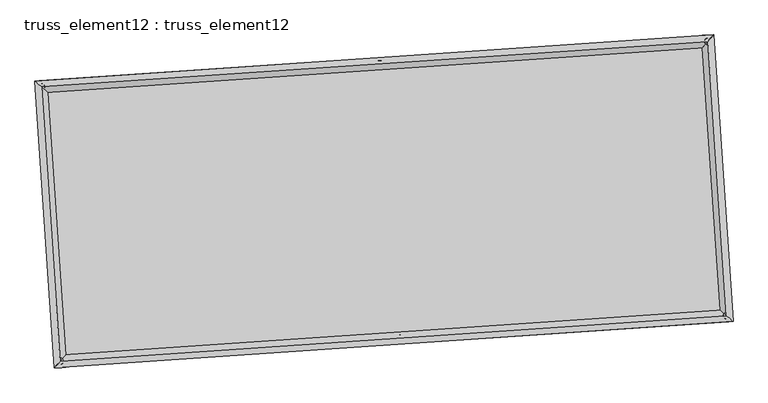
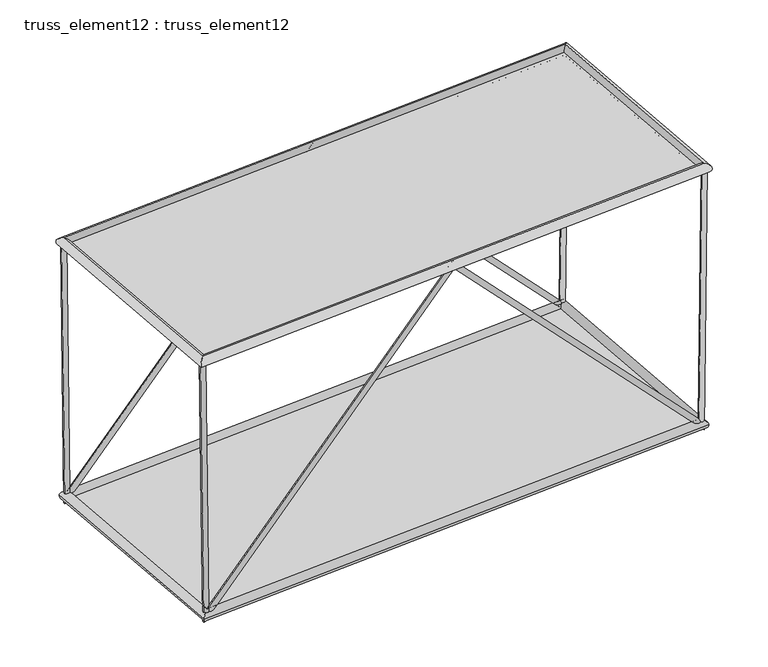
"""IFC4 building model written with IfcOpenShell, lengths in millimetres: plate geometry, truss_element12 : truss_element12."""

import ifcopenshell
import ifcopenshell.guid

model = None  # the IFC model being written
_history = None  # IfcOwnerHistory: only IFC2X3 demands one
_inside = {}  # id of a spatial element -> (the spatial element, [elements in it])
_under = {}  # id of a project, library or spatial element -> (it, [spatial elements below it])
_declared = {}  # id of a project -> (the project, [libraries it declares])
_typed = {}  # id of a type object -> (the type object, [elements of that type])
_made_of = {}  # id of a material, layer set ... -> (it, [elements and type objects made of it])


def new_model(schema):
    """Start an empty IFC model of exactly this schema.

    Asked for "IFC4X3", IfcOpenShell would pick the latest addendum, in which some entities
    have other attributes; the version numbers below select the first issue.
    IFC2X3 requires an IfcOwnerHistory on every rooted entity: one is made here for all.
    """
    global model, _history
    if schema == "IFC4X3":
        model = ifcopenshell.file(schema_version=(4, 3, 0, 0))
    else:
        model = ifcopenshell.file(schema=schema)
    _inside.clear()
    _under.clear()
    _declared.clear()
    _typed.clear()
    _made_of.clear()
    _history = None
    if model.schema == "IFC2X3":
        org = make("IfcOrganization", Name="unknown")
        user = make(
            "IfcPersonAndOrganization",
            ThePerson=make("IfcPerson", FamilyName="unknown"),
            TheOrganization=org,
        )
        app = make(
            "IfcApplication",
            ApplicationDeveloper=org,
            Version="unknown",
            ApplicationFullName="unknown",
            ApplicationIdentifier="unknown",
        )
        _history = make(
            "IfcOwnerHistory",
            OwningUser=user,
            OwningApplication=app,
            ChangeAction="ADDED",
            CreationDate=0,
        )
    return model


def make(cls, **values):
    """One entity of the class cls with the attributes given. An attribute that is None is left unset."""
    return model.create_entity(
        cls, **{name: value for name, value in values.items() if value is not None}
    )


def rooted(cls, **values):
    """An entity with a GlobalId (a new one), such as an element, a storey or a relation."""
    return make(cls, GlobalId=ifcopenshell.guid.new(), OwnerHistory=_history, **values)


def si_unit(unit_type, name, prefix=None):
    """IfcSIUnit, for example si_unit("LENGTHUNIT", "METRE", prefix="MILLI")."""
    return make("IfcSIUnit", UnitType=unit_type, Prefix=prefix, Name=name)


def assignment(units):
    """IfcUnitAssignment: the units of a project."""
    return None if units is None else make("IfcUnitAssignment", Units=units)


def point(xyz):
    """IfcCartesianPoint."""
    return None if xyz is None else make("IfcCartesianPoint", Coordinates=xyz)


def direction(xyz):
    """IfcDirection."""
    return None if xyz is None else make("IfcDirection", DirectionRatios=xyz)


def frame(location, z_axis=None, x_axis=None):
    """IfcAxis2Placement3D, a coordinate frame: its origin and axes. An axis left out is left unset."""
    return make(
        "IfcAxis2Placement3D",
        Location=point(location),
        Axis=direction(z_axis),
        RefDirection=direction(x_axis),
    )


def origin():
    """The frame at (0, 0, 0) with its axes left unset."""
    return frame((0.0, 0.0, 0.0))


def origin_with_axes():
    """The frame at (0, 0, 0) with the z axis (0, 0, 1) and the x axis (1, 0, 0) written out."""
    return frame((0.0, 0.0, 0.0), z_axis=(0.0, 0.0, 1.0), x_axis=(1.0, 0.0, 0.0))


def place(relative_to, where):
    """IfcLocalPlacement: puts the frame where relative to a parent placement (None: the world)."""
    return make(
        "IfcLocalPlacement", PlacementRelTo=relative_to, RelativePlacement=where
    )


def context(
    kind, dimensions, precision=None, world=None, true_north=None, identifier=None
):
    """IfcGeometricRepresentationContext, for example the 3D "Model" context."""
    return make(
        "IfcGeometricRepresentationContext",
        ContextIdentifier=identifier,
        ContextType=kind,
        CoordinateSpaceDimension=dimensions,
        Precision=precision,
        WorldCoordinateSystem=world,
        TrueNorth=true_north,
    )


def project(units=None, contexts=None):
    """IfcProject with its units and contexts."""
    return rooted(
        "IfcProject",
        Name="project",
        RepresentationContexts=contexts,
        UnitsInContext=assignment(units),
    )


def spatial(cls, under=None, at=None, **own):
    """A site, building, storey or space (cls), placed at a placement, below another one or the project."""
    s = rooted(cls, ObjectPlacement=at, **own)
    if under is not None:
        _under.setdefault(under.id(), (under, []))[1].append(s)
    return s


def polyline(points):
    """IfcPolyline through the points."""
    return make("IfcPolyline", Points=[point(p) for p in points])


def circle_curve(where, radius):
    """IfcCircle in the frame where."""
    return make("IfcCircle", Position=where, Radius=radius)


def ellipse_curve(where, semi_axis1, semi_axis2):
    """IfcEllipse in the frame where."""
    return make(
        "IfcEllipse", Position=where, SemiAxis1=semi_axis1, SemiAxis2=semi_axis2
    )


def outline(outer, holes=None, kind="AREA"):
    """IfcArbitraryClosedProfileDef: a profile drawn as a closed curve; with holes, ...WithVoids."""
    if holes is None:
        return make("IfcArbitraryClosedProfileDef", ProfileType=kind, OuterCurve=outer)
    return make(
        "IfcArbitraryProfileDefWithVoids",
        ProfileType=kind,
        OuterCurve=outer,
        InnerCurves=holes,
    )


def extrude(swept, where, along, depth):
    """IfcExtrudedAreaSolid: the profile swept, set in the frame where, extruded along a direction by depth."""
    return make(
        "IfcExtrudedAreaSolid",
        SweptArea=swept,
        Position=where,
        ExtrudedDirection=direction(along),
        Depth=depth,
    )


def shape(context_of_items, identifier, shape_type, items):
    """IfcShapeRepresentation: the items that make up one representation, for example the "Body"."""
    return make(
        "IfcShapeRepresentation",
        ContextOfItems=context_of_items,
        RepresentationIdentifier=identifier,
        RepresentationType=shape_type,
        Items=items,
    )


def source(mapping_origin, context_of_items, identifier, shape_type, items):
    """IfcRepresentationMap: a shape defined once, which mapped items show again and again."""
    return make(
        "IfcRepresentationMap",
        MappingOrigin=mapping_origin,
        MappedRepresentation=shape(context_of_items, identifier, shape_type, items),
    )


def transform(
    local_origin,
    x_axis=None,
    y_axis=None,
    z_axis=None,
    scale=None,
    scale2=None,
    scale3=None,
    uniform=True,
):
    """IfcCartesianTransformationOperator3D, or its non-uniform kind. x_axis, y_axis, z_axis: its Axis1, 2, 3."""
    if uniform:
        return make(
            "IfcCartesianTransformationOperator3D",
            Axis1=direction(x_axis),
            Axis2=direction(y_axis),
            LocalOrigin=point(local_origin),
            Scale=scale,
            Axis3=direction(z_axis),
        )
    return make(
        "IfcCartesianTransformationOperator3DnonUniform",
        Axis1=direction(x_axis),
        Axis2=direction(y_axis),
        LocalOrigin=point(local_origin),
        Scale=scale,
        Axis3=direction(z_axis),
        Scale2=scale2,
        Scale3=scale3,
    )


def mapped(mapping_source, mapping_target):
    """IfcMappedItem: shows the shape of a source again, moved by a transform."""
    return make(
        "IfcMappedItem", MappingSource=mapping_source, MappingTarget=mapping_target
    )


def made_of(thing, what):
    """Note that an element or type object is made of a material, layer set ...; save() writes the relation."""
    if what is not None:
        _made_of.setdefault(what.id(), (what, []))[1].append(thing)
    return thing


def element(
    cls,
    number,
    at=None,
    inside=None,
    cuts=None,
    type_object=None,
    material=None,
    context=None,
    identifier="Body",
    shape_type=None,
    held_by="IfcProductDefinitionShape",
    body=None,
    shapes=None,
    **own,
):
    """One element of the class cls, such as IfcWall. Its Tag is "e" and its number.

    at: its placement. inside: the storey or other place that contains it. cuts: it is an
    opening in that element (IfcRelVoidsElement). A single representation is given by context,
    identifier, shape_type and body (its items); several are given by shapes. held_by: the class
    of the entity that holds the representations. save() writes the other relations.
    """
    e = rooted(cls, Tag="e%d" % number, ObjectPlacement=at, **own)
    if body is not None:
        shapes = [shape(context, identifier, shape_type, body)]
    if shapes is not None:
        e.Representation = make(held_by, Representations=shapes)
    if inside is not None:
        _inside.setdefault(inside.id(), (inside, []))[1].append(e)
    if cuts is not None:
        rooted(
            "IfcRelVoidsElement", RelatingBuildingElement=cuts, RelatedOpeningElement=e
        )
    if type_object is not None:
        _typed.setdefault(type_object.id(), (type_object, []))[1].append(e)
    return made_of(e, material)


def aggregate(whole, parts):
    """IfcRelAggregates: a whole, such as a stair, and the parts it consists of."""
    return rooted("IfcRelAggregates", RelatingObject=whole, RelatedObjects=parts)


def save(model, path):
    """Write the relations noted so far, then the file.

    IfcRelAggregates (storeys below a building ...), IfcRelContainedInSpatialStructure (elements
    in a storey), IfcRelDefinesByType, IfcRelAssociatesMaterial and IfcRelDeclares: one each for
    every whole, place, type object, material and project.
    """
    for whole, parts in _under.values():
        aggregate(whole, parts)
    for where, things in _inside.values():
        rooted(
            "IfcRelContainedInSpatialStructure",
            RelatedElements=things,
            RelatingStructure=where,
        )
    for kind, things in _typed.values():
        rooted("IfcRelDefinesByType", RelatedObjects=things, RelatingType=kind)
    for what, things in _made_of.values():
        rooted("IfcRelAssociatesMaterial", RelatedObjects=things, RelatingMaterial=what)
    for by, libraries in _declared.values():
        rooted("IfcRelDeclares", RelatingContext=by, RelatedDefinitions=libraries)
    model.write(path)


def plane_surface(at):
    """IfcPlane: the flat surface through the origin of the frame at, square to its z axis."""
    return make("IfcPlane", Position=at)


def cylinder_surface(at, radius):
    """IfcCylindricalSurface: all points at the distance radius from the z axis of the frame at."""
    return make("IfcCylindricalSurface", Position=at, Radius=radius)


def advanced_brep(points, edges, surfaces, faces):
    """IfcAdvancedBrep: a solid bounded by faces that lie on surfaces and meet in shared edges.

    An edge is (start, end): straight between two places in points (the first is 0);
    or (start, end, curve); or (start, end, curve, False) where it runs against its curve.
    A face is (place in surfaces, loops), or (place, loops, False) where it looks against
    its surface's normal. A loop lists edges by number (the first is 1), with a minus sign
    where the edge is run from its end to its start. The first loop is the outer one.
    """
    corners = [point(p) for p in points]
    vertices = [make("IfcVertexPoint", VertexGeometry=c) for c in corners]
    made = []
    for start, end, *more in edges:
        made.append(
            make(
                "IfcEdgeCurve",
                EdgeStart=vertices[start],
                EdgeEnd=vertices[end],
                EdgeGeometry=more[0] if more else make("IfcPolyline", Points=[corners[start], corners[end]]),
                SameSense=more[1] if len(more) > 1 else True,
            )
        )
    hull = []
    for where, loops, *sense in faces:
        bounds = []
        for j, loop in enumerate(loops):
            ring = [make("IfcOrientedEdge", EdgeElement=made[abs(k) - 1], Orientation=k > 0) for k in loop]
            bounds.append(
                make(
                    "IfcFaceOuterBound" if j == 0 else "IfcFaceBound",
                    Bound=make("IfcEdgeLoop", EdgeList=ring),
                    Orientation=True,
                )
            )
        hull.append(make("IfcAdvancedFace", Bounds=bounds, FaceSurface=surfaces[where], SameSense=sense[0] if sense else True))
    return make("IfcAdvancedBrep", Outer=make("IfcClosedShell", CfsFaces=hull))


def truss_element12_truss_element12_2c86acb7(model_context):
    return source(origin(), model_context, "Body", "SolidModel", [
        advanced_brep(
        [(-3728.3550112, 2271.9000693, 5000.230225), (-3827.45033, 2258.5393422, 4998.9618576), (-3666.4925131, 2276.1182379, 122.5885244), (-3762.4943697, 2262.9684422, -122.5885244), (1063.1473442, 2598.6144007, 5071.7241818), (1063.6040901, 2592.0417504, 4927.4822409), (5793.903749, 2921.1866967, 122.5964773), (5890.857228, 2921.1937918, -122.5964773), (5854.658099, 2925.3293049, 5000.2332074), (5954.6501108, 2925.543586, 4998.9875555)],
        [
            (0, 1, circle_curve(frame((-3777.9026706, 2265.2197058, 4999.5960413), z_axis=(-0.012681845830498275, -0.0008647268589742656, 0.9999192082532422), x_axis=(-0.13360744533254773, 0.991033979828119, -0.0008374829847137765)), 50.0)),
            (1, 0, circle_curve(frame((-3777.9026706, 2265.2197058, 4999.5960413), z_axis=(-0.012681845830498275, -0.0008647268589742656, 0.9999192082532422), x_axis=(-0.13360744533254773, 0.991033979828119, -0.0008374829847137765)), 50.0)),
            (0, 2),
            (2, 3, ellipse_curve(frame((-3714.4934414, 2269.54334, 0.0), z_axis=(-0.9281379125811652, -0.06328619607639939, 0.3668172196280557), x_axis=(0.36596744941726267, 0.02495392920324594, 0.9302930330730971)), 132.0610358, 50.0)),
            (3, 1),
            (3, 2, ellipse_curve(frame((-3714.4934414, 2269.54334, 0.0), z_axis=(-0.9281379125811652, -0.06328619607639939, 0.3668172196280557), x_axis=(0.36596744941726267, 0.02495392920324594, 0.9302930330730971)), 132.0610358, 50.0)),
            (2, 4),
            (4, 5, ellipse_curve(frame((1063.3757172, 2595.3280756, 4999.6032114), z_axis=(-0.99768339431723, -0.068028238108855, -5.9358703528731525e-05), x_axis=(5.922119292306359e-05, 4.038068026292035e-06, -0.9999999982382721)), 72.2780144, 50.0)),
            (5, 3),
            (5, 4, ellipse_curve(frame((1063.3757172, 2595.3280756, 4999.6032114), z_axis=(-0.99768339431723, -0.068028238108855, -5.9358703528731525e-05), x_axis=(5.922119292306359e-05, 4.038068026292035e-06, -0.9999999982382721)), 72.2780144, 50.0)),
            (4, 6),
            (6, 7, ellipse_curve(frame((5842.3804885, 2921.1902443, 0.0), z_axis=(-0.9280745157714422, -0.06328187328893672, -0.3669783340861503), x_axis=(-0.3661281906369709, -0.02496488953598652, 0.9302294890570573)), 132.0786249, 50.0)),
            (7, 5),
            (7, 6, ellipse_curve(frame((5842.3804885, 2921.1902443, 0.0), z_axis=(-0.9280745157714422, -0.06328187328893672, -0.3669783340861503), x_axis=(-0.3661281906369709, -0.02496488953598652, 0.9302294890570573)), 132.0786249, 50.0)),
            (8, 9, circle_curve(frame((5904.6541049, 2925.4364454, 4999.6103815), z_axis=(0.012454723282468173, 0.0008492402357941579, 0.9999220762934375), x_axis=(-0.002153222592044798, 0.9999973435725115, -0.0008224842793232085)), 50.0)),
            (9, 8, circle_curve(frame((5904.6541049, 2925.4364454, 4999.6103815), z_axis=(0.012454723282468173, 0.0008492402357941579, 0.9999220762934375), x_axis=(-0.002153222592044798, 0.9999973435725115, -0.0008224842793232085)), 50.0)),
            (6, 8),
            (9, 7),
        ],
        [
            plane_surface(frame((-3777.9026706, 2315.2196871, 4999.6392811), z_axis=(-0.012681845830499536, -0.000864726858973905, 0.9999192082532424), x_axis=(0.9999195821596513, -1.0967214670642997e-05, 0.012681841088294742))),
            cylinder_surface(frame((-3777.9026706, 2265.2197058, 4999.5960413), z_axis=(-0.012681845830498278, -0.0008647268589742659, 0.9999192082532424), x_axis=(-0.13360744533254773, 0.991033979828119, -0.0008374829847137765)), 50.0),
            cylinder_surface(frame((-3714.4934414, 2269.54334, 0.0), z_axis=(-0.6901279623524452, -0.04705720233082468, -0.7221558109494499), x_axis=(-0.020411445780293115, 0.9987523847393089, -0.04557462955089897)), 50.0),
            cylinder_surface(frame((1063.3757172, 2595.3280756, 4999.6032114), z_axis=(-0.6902134913462256, -0.04706303422778687, 0.7220736854178583), x_axis=(-0.11534401236489931, 0.9922792938963748, -0.04558027770953044)), 50.0),
            plane_surface(frame((5904.6541049, 2875.4364635, 4999.6528468), z_axis=(0.012454723282466664, 0.0008492402357928526, 0.9999220762934377), x_axis=(0.9999224369259634, -1.0577872590289415e-05, -0.012454718790539939))),
            cylinder_surface(frame((5842.3804885, 2921.1902443, 0.0), z_axis=(-0.012454723282468173, -0.0008492402357941579, -0.9999220762934375), x_axis=(-0.002153222592044798, 0.9999973435725115, -0.0008224842793232085)), 50.0),
        ],
        [
            (0, [[1, 2]]),
            (1, [[-1, 3, 4, 5]]),
            (1, [[-2, -5, 6, -3]]),
            (2, [[-4, 7, 8, 9]]),
            (2, [[-6, -9, 10, -7]]),
            (3, [[-8, 11, 12, 13]]),
            (3, [[-10, -13, 14, -11]]),
            (4, [[15, 16]]),
            (5, [[-12, 17, -16, 18]]),
            (5, [[-14, -18, -15, -17]]),
        ],
    ),
        advanced_brep(
        [(-3456.2420582, -1718.833515, 5000.230225), (-3555.3373771, -1732.1942421, 4998.9618576), (-3394.3795602, -1714.6153464, 122.5885244), (-3490.3814168, -1727.7651421, -122.5885244), (1335.2602971, -1392.1191836, 5071.7241818), (1335.7170431, -1398.6918339, 4927.4822409), (6066.016702, -1069.5468876, 122.5964773), (6162.9701809, -1069.5397925, -122.5964773), (6126.7710519, -1065.4042794, 5000.2332074), (6226.7630638, -1065.1899983, 4998.9875555)],
        [
            (0, 1, circle_curve(frame((-3505.7897177, -1725.5138785, 4999.5960413), z_axis=(-0.012681845830497715, -0.0008647268589742125, 0.9999192082532423), x_axis=(-0.13360744533254784, 0.991033979828119, -0.0008374829847137556)), 50.0)),
            (1, 0, circle_curve(frame((-3505.7897177, -1725.5138785, 4999.5960413), z_axis=(-0.012681845830497715, -0.0008647268589742125, 0.9999192082532423), x_axis=(-0.13360744533254784, 0.991033979828119, -0.0008374829847137556)), 50.0)),
            (0, 2),
            (2, 3, ellipse_curve(frame((-3442.3804885, -1721.1902443, 0.0), z_axis=(-0.9281379125811646, -0.06328619607639936, 0.36681721962805663), x_axis=(0.3659674494172635, 0.02495392920324602, 0.930293033073097)), 132.0610358, 50.0)),
            (3, 1),
            (3, 2, ellipse_curve(frame((-3442.3804885, -1721.1902443, 0.0), z_axis=(-0.9281379125811646, -0.06328619607639936, 0.36681721962805663), x_axis=(0.3659674494172635, 0.02495392920324602, 0.930293033073097)), 132.0610358, 50.0)),
            (2, 4),
            (4, 5, ellipse_curve(frame((1335.4886701, -1395.4055087, 4999.6032114), z_axis=(-0.9976833943172299, -0.06802823810885503, -5.935870352808952e-05), x_axis=(5.922119292244865e-05, 4.03806802626321e-06, -0.9999999982382721)), 72.2780144, 50.0)),
            (5, 3),
            (5, 4, ellipse_curve(frame((1335.4886701, -1395.4055087, 4999.6032114), z_axis=(-0.9976833943172299, -0.06802823810885503, -5.935870352808952e-05), x_axis=(5.922119292244865e-05, 4.03806802626321e-06, -0.9999999982382721)), 72.2780144, 50.0)),
            (4, 6),
            (6, 7, ellipse_curve(frame((6114.4934414, -1069.54334, 0.0), z_axis=(-0.928074515771442, -0.06328187328893677, -0.3669783340861506), x_axis=(-0.3661281906369714, -0.024964889535986565, 0.9302294890570572)), 132.0786249, 50.0)),
            (7, 5),
            (7, 6, ellipse_curve(frame((6114.4934414, -1069.54334, 0.0), z_axis=(-0.928074515771442, -0.06328187328893677, -0.3669783340861506), x_axis=(-0.3661281906369714, -0.024964889535986565, 0.9302294890570572)), 132.0786249, 50.0)),
            (8, 9, circle_curve(frame((6176.7670578, -1065.2971389, 4999.6103815), z_axis=(0.012454723282467507, 0.0008492402357941209, 0.9999220762934375), x_axis=(-0.0021532225920447086, 0.9999973435725115, -0.0008224842793231741)), 50.0)),
            (9, 8, circle_curve(frame((6176.7670578, -1065.2971389, 4999.6103815), z_axis=(0.012454723282467507, 0.0008492402357941209, 0.9999220762934375), x_axis=(-0.0021532225920447086, 0.9999973435725115, -0.0008224842793231741)), 50.0)),
            (6, 8),
            (9, 7),
        ],
        [
            plane_surface(frame((-3505.7897177, -1675.5138972, 4999.6392811), z_axis=(-0.012681845830499536, -0.000864726858973898, 0.9999192082532424), x_axis=(0.9999195821596513, -1.0967214670642997e-05, 0.012681841088294742))),
            cylinder_surface(frame((-3505.7897177, -1725.5138785, 4999.5960413), z_axis=(-0.012681845830497715, -0.0008647268589742125, 0.9999192082532423), x_axis=(-0.13360744533254784, 0.991033979828119, -0.0008374829847137556)), 50.0),
            cylinder_surface(frame((-3442.3804885, -1721.1902443, 0.0), z_axis=(-0.6901279623524461, -0.047057202330824756, -0.722155810949449), x_axis=(-0.020411445780293143, 0.9987523847393089, -0.045574629550899075)), 50.0),
            cylinder_surface(frame((1335.4886701, -1395.4055087, 4999.6032114), z_axis=(-0.6902134913462256, -0.047063034227786904, 0.7220736854178583), x_axis=(-0.11534401236489945, 0.9922792938963748, -0.045580277709530506)), 50.0),
            plane_surface(frame((6176.7670578, -1115.2971208, 4999.6528468), z_axis=(0.012454723282466664, 0.0008492402357928471, 0.9999220762934377), x_axis=(0.9999224369259634, -1.0577872589401237e-05, -0.012454718790539939))),
            cylinder_surface(frame((6114.4934414, -1069.54334, 0.0), z_axis=(-0.012454723282467507, -0.0008492402357941209, -0.9999220762934375), x_axis=(-0.0021532225920447086, 0.9999973435725115, -0.0008224842793231741)), 50.0),
        ],
        [
            (0, [[1, 2]]),
            (1, [[-1, 3, 4, 5]]),
            (1, [[-2, -5, 6, -3]]),
            (2, [[-4, 7, 8, 9]]),
            (2, [[-6, -9, 10, -7]]),
            (3, [[-8, 11, 12, 13]]),
            (3, [[-10, -13, 14, -11]]),
            (4, [[15, 16]]),
            (5, [[-12, 17, -16, 18]]),
            (5, [[-14, -18, -15, -17]]),
        ],
    ),
        advanced_brep(
        [(-3505.7859545, -1725.5097077, 4909.5960414), (-3505.7934808, -1725.5180494, 5089.5960412), (-3777.906965, 2265.2233272, 5089.5960412), (-3777.8983761, 2265.2160844, 4909.5960414), (5904.6576027, 2925.4405981, 5089.6103814), (5904.6506071, 2925.4322927, 4909.6103815), (6176.7710869, -1065.3007784, 5089.6103814), (6176.7630287, -1065.2934994, 4909.6103815)],
        [
            (0, 1, ellipse_curve(frame((-3505.7897177, -1725.5138785, 4999.5960413), z_axis=(-0.7535719234046869, 0.6573654662781344, -1.0448234971291915e-06), x_axis=(-0.6573654662773117, -0.7535719234054046, -1.0448235032548692e-06)), 127.2792206, 90.0)),
            (1, 2),
            (2, 3, ellipse_curve(frame((-3777.9026706, 2265.2197058, 4999.5960413), z_axis=(-0.6573654662773116, -0.7535719234054046, -1.0448235045172827e-06), x_axis=(0.7535719234046869, -0.6573654662781343, 1.0448234983916052e-06)), 127.2792206, 90.0)),
            (3, 0),
            (1, 0, ellipse_curve(frame((-3505.7897177, -1725.5138785, 4999.5960413), z_axis=(-0.7535719234046869, 0.6573654662781344, -1.0448234971291915e-06), x_axis=(-0.6573654662773117, -0.7535719234054046, -1.0448235032548692e-06)), 127.2792206, 90.0)),
            (3, 2, ellipse_curve(frame((-3777.9026706, 2265.2197058, 4999.5960413), z_axis=(-0.6573654662773116, -0.7535719234054046, -1.0448235045172827e-06), x_axis=(0.7535719234046869, -0.6573654662781343, 1.0448234983916052e-06)), 127.2792206, 90.0)),
            (2, 4),
            (4, 5, ellipse_curve(frame((5904.6541049, 2925.4364454, 4999.6103815), z_axis=(-0.7535719234046876, 0.6573654662781336, -1.0448234953288471e-06), x_axis=(-0.6573654662773109, -0.7535719234054052, -1.0448235075800405e-06)), 127.2792206, 90.0)),
            (5, 3),
            (5, 4, ellipse_curve(frame((5904.6541049, 2925.4364454, 4999.6103815), z_axis=(-0.7535719234046876, 0.6573654662781336, -1.0448234953288471e-06), x_axis=(-0.6573654662773109, -0.7535719234054052, -1.0448235075800405e-06)), 127.2792206, 90.0)),
            (4, 6),
            (6, 7, ellipse_curve(frame((6176.7670578, -1065.2971389, 4999.6103815), z_axis=(0.657365466277311, 0.753571923405405, 1.044823506317627e-06), x_axis=(-0.7535719234046873, 0.6573654662781341, -1.0448234940664328e-06)), 127.2792206, 90.0)),
            (7, 5),
            (7, 6, ellipse_curve(frame((6176.7670578, -1065.2971389, 4999.6103815), z_axis=(0.657365466277311, 0.753571923405405, 1.044823506317627e-06), x_axis=(-0.7535719234046873, 0.6573654662781341, -1.0448234940664328e-06)), 127.2792206, 90.0)),
            (6, 1),
            (0, 7),
        ],
        [
            cylinder_surface(frame((-3505.7897177, -1725.5138785, 4999.5960413), z_axis=(0.06802823822869937, -0.9976833960748767, 0.0), x_axis=(-0.997683395070632, -0.06802823816022374, -4.486817461283446e-05)), 90.0),
            cylinder_surface(frame((-3777.9026706, 2265.2197058, 4999.5960413), z_axis=(-0.9976833960737876, -0.06802823822862634, -1.47760356604302e-06), x_axis=(-0.06802823810069528, 0.9976833951400482, -4.339057104385098e-05)), 90.0),
            cylinder_surface(frame((5904.6541049, 2925.4364454, 4999.6103815), z_axis=(-0.06802823822870101, 0.9976833960748767, 0.0), x_axis=(0.997683395198563, 0.06802823816894851, -4.19129674878619e-05)), 90.0),
            cylinder_surface(frame((6176.7670578, -1065.2971389, 4999.6103815), z_axis=(0.9976833960737875, 0.06802823822862625, 1.4776035642576973e-06), x_axis=(0.06802823822862625, -0.997683395131325, -4.339057105939159e-05)), 90.0),
        ],
        [
            (0, [[1, 2, 3, 4]]),
            (0, [[5, -4, 6, -2]]),
            (1, [[-3, 7, 8, 9]]),
            (1, [[-6, -9, 10, -7]]),
            (2, [[-8, 11, 12, 13]]),
            (2, [[-10, -13, 14, -11]]),
            (3, [[-12, 15, -1, 16]]),
            (3, [[-14, -16, -5, -15]]),
        ],
    ),
        advanced_brep(
        [(-3358.7115243, -1625.2761972, 0.0), (-3526.0494527, -1817.1042913, 0.0), (-3810.4074885, 2353.2123043, 0.0), (-3618.5793943, 2185.8743758, 0.0), (5926.0494527, 3017.1042913, 0.0), (5758.7115243, 2825.2761972, 0.0), (6210.4074885, -1153.2123043, 0.0), (6018.5793943, -985.8743758, 0.0)],
        [
            (0, 1, ellipse_curve(frame((-3442.3804885, -1721.1902443, 0.0), z_axis=(-0.753571923405458, 0.6573654662780806, 0.0), x_axis=(-0.6573654662780806, -0.753571923405458, 0.0)), 127.2792206, 90.0)),
            (1, 2),
            (2, 3, ellipse_curve(frame((-3714.4934414, 2269.54334, 0.0), z_axis=(-0.6573654662780806, -0.753571923405458, 0.0), x_axis=(0.7535719234054579, -0.6573654662780809, 0.0)), 127.2792206, 90.0)),
            (3, 0),
            (1, 0, ellipse_curve(frame((-3442.3804885, -1721.1902443, 0.0), z_axis=(-0.753571923405458, 0.6573654662780806, 0.0), x_axis=(-0.6573654662780806, -0.753571923405458, 0.0)), 127.2792206, 90.0)),
            (3, 2, ellipse_curve(frame((-3714.4934414, 2269.54334, 0.0), z_axis=(-0.6573654662780806, -0.753571923405458, 0.0), x_axis=(0.7535719234054579, -0.6573654662780809, 0.0)), 127.2792206, 90.0)),
            (2, 4),
            (4, 5, ellipse_curve(frame((5842.3804885, 2921.1902443, 0.0), z_axis=(-0.7535719234054586, 0.6573654662780799, 0.0), x_axis=(-0.6573654662780801, -0.7535719234054584, 0.0)), 127.2792206, 90.0)),
            (5, 3),
            (5, 4, ellipse_curve(frame((5842.3804885, 2921.1902443, 0.0), z_axis=(-0.7535719234054586, 0.6573654662780799, 0.0), x_axis=(-0.6573654662780801, -0.7535719234054584, 0.0)), 127.2792206, 90.0)),
            (4, 6),
            (6, 7, ellipse_curve(frame((6114.4934414, -1069.54334, 0.0), z_axis=(0.6573654662780799, 0.7535719234054586, 0.0), x_axis=(-0.7535719234054586, 0.6573654662780799, 0.0)), 127.2792206, 90.0)),
            (7, 5),
            (7, 6, ellipse_curve(frame((6114.4934414, -1069.54334, 0.0), z_axis=(0.6573654662780799, 0.7535719234054586, 0.0), x_axis=(-0.7535719234054586, 0.6573654662780799, 0.0)), 127.2792206, 90.0)),
            (6, 1),
            (0, 7),
        ],
        [
            cylinder_surface(frame((-3442.3804885, -1721.1902443, 0.0), z_axis=(0.06802823822870088, -0.9976833960748768, 0.0), x_axis=(-0.9976833960748768, -0.06802823822870088, 0.0)), 90.0),
            cylinder_surface(frame((-3714.4934414, 2269.54334, 0.0), z_axis=(-0.9976833960748767, -0.06802823822870208, 0.0), x_axis=(-0.06802823822870208, 0.9976833960748767, 0.0)), 90.0),
            cylinder_surface(frame((5842.3804885, 2921.1902443, 0.0), z_axis=(-0.06802823822870274, 0.9976833960748765, 0.0), x_axis=(0.9976833960748765, 0.06802823822870274, 0.0)), 90.0),
            cylinder_surface(frame((6114.4934414, -1069.54334, 0.0), z_axis=(0.9976833960748767, 0.06802823822870205, 0.0), x_axis=(0.06802823822870205, -0.9976833960748767, 0.0)), 90.0),
        ],
        [
            (0, [[1, 2, 3, 4]]),
            (0, [[5, -4, 6, -2]]),
            (1, [[-3, 7, 8, 9]]),
            (1, [[-6, -9, 10, -7]]),
            (2, [[-8, 11, 12, 13]]),
            (2, [[-10, -13, 14, -11]]),
            (3, [[-12, 15, -1, 16]]),
            (3, [[-14, -16, -5, -15]]),
        ],
    ),
        extrude(outline(polyline([(-3442.3804885, -1721.1902443), (-3714.4934414, 2269.54334), (5842.3804885, 2921.1902443), (6114.4934414, -1069.54334), (-3442.3804885, -1721.1902443)])), origin_with_axes(), (0.0, 0.0, 1.0), 20.0),
        extrude(outline(polyline([(-1999.9999999, 4852.5197541), (2000.0000001, 4852.5197541), (2000.0, -4852.5197541), (-2000.0, -4852.5197541), (-1999.9999999, 4852.5197541)])), frame((1199.4321936, 599.9612834, 4999.6032114), z_axis=(-1.474180543527448e-06, -1.0051877171978412e-07, 0.9999999999989084), x_axis=(-0.06802823822870088, 0.9976833960748767, 0.0)), (0.0, 0.0, 1.0), 20.0),
    ])


if __name__ == "__main__":
    model = new_model("IFC4")
    model_context = context("Model", 3, world=origin())
    ifc_project = project(units=[si_unit("LENGTHUNIT", "METRE", prefix="MILLI")], contexts=[model_context])
    site = spatial("IfcSite", under=ifc_project)
    building = spatial("IfcBuilding", under=site)
    placement = place(None, origin())
    truss_element12_truss_element12_shape = truss_element12_truss_element12_2c86acb7(model_context)
    element("IfcPlate", 1, ObjectType="truss_element12 : truss_element12", at=placement, inside=building, context=model_context, shape_type="MappedRepresentation", body=[
        mapped(truss_element12_truss_element12_shape, transform((0.0, 0.0, 0.0), x_axis=(1.0, 0.0, 0.0), y_axis=(0.0, 1.0, 0.0), z_axis=(0.0, 0.0, 1.0))),
    ])
    save(model, "model.ifc")

# Revit data of these elements
# Type "truss_element12 : truss_element12"
#   steellbar1 = 90 mm
#   steelbar2 = 50 mm
#   offset1 = 5000 mm
#   M = Default Roof
# Element 1 (IfcPlate, "truss_element12 : truss_element12")
#   Materials on its faces: "Default Roof"
# Materials
#   "Default Roof": class "Miscellaneous", colour RGB 0 127 0, transparency 0, Comments = "Rendering appearance not upgraded Rendering appearance not upgraded ", Cost = 0
